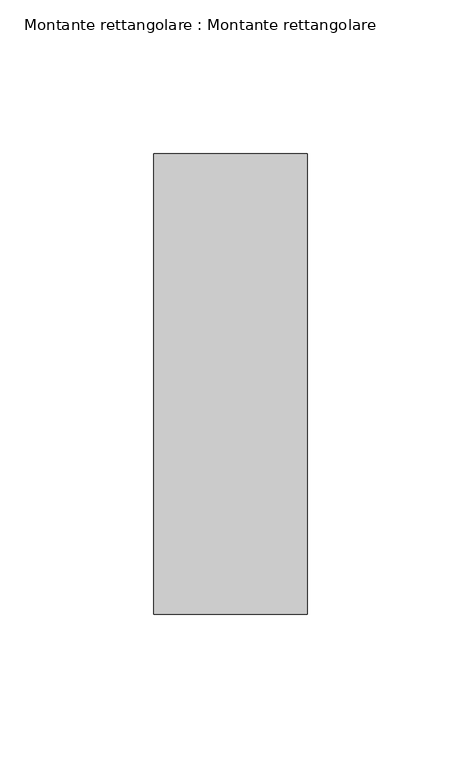
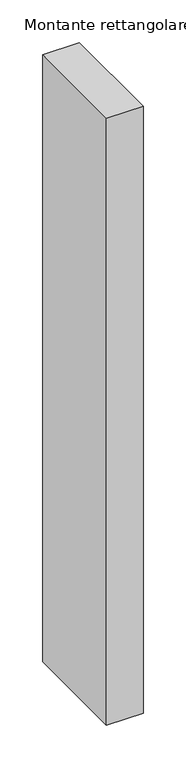
"""IFC4 building model written with IfcOpenShell, lengths in millimetres: member geometry, Montante rettangolare : Montante rettangolare."""

from ifc_helpers import new_model, si_unit, frame, origin, place, context, project, spatial, polyline, outline, extrude, source, transform, mapped, element, save


def montante_rettangolare_montante_rettangolare_c57c7bcc(model_context):
    return source(origin(), model_context, "Body", "SweptSolid", [
        extrude(outline(polyline([(0.0, 75.0), (0.0, -75.0), (-50.0, -75.0), (-50.0, 75.0), (0.0, 75.0)])), frame((0.0, 0.0, -870.0), z_axis=(0.0, 0.0, 1.0), x_axis=(1.0, 0.0, 0.0)), (0.0, 0.0, 1.0), 870.0),
    ])


if __name__ == "__main__":
    model = new_model("IFC4")
    model_context = context("Model", 3, world=origin())
    ifc_project = project(units=[si_unit("LENGTHUNIT", "METRE", prefix="MILLI")], contexts=[model_context])
    site = spatial("IfcSite", under=ifc_project)
    building = spatial("IfcBuilding", under=site)
    placement = place(None, origin())
    montante_rettangolare_montante_rettangolare_shape = montante_rettangolare_montante_rettangolare_c57c7bcc(model_context)
    element("IfcMember", 1, ObjectType="Montante rettangolare : Montante rettangolare", at=placement, inside=building, context=model_context, shape_type="MappedRepresentation", body=[
        mapped(montante_rettangolare_montante_rettangolare_shape, transform((0.0, 0.0, 0.0), x_axis=(1.0, 0.0, 0.0), y_axis=(0.0, 1.0, 0.0), z_axis=(0.0, 0.0, 1.0))),
    ])
    save(model, "model.ifc")

# Revit data of these elements
# Type "Montante rettangolare : Montante rettangolare"
#   built-in parameter 1007304 = 0.492126 (stored number, unit not read)
#   built-in parameter 1007301 = 0.082021 (stored number, unit not read)
#   built-in parameter 1007300 = 0.082021 (stored number, unit not read)
# Element 1 (IfcMember, "Montante rettangolare : Montante rettangolare")
#   Materials on its faces: "Acciaio"
# Materials
#   "Acciaio": class "Metallo", colour RGB 247 247 247, transparency 0, Description = "Acciaio, finitura zigrinata", Cost = 0
